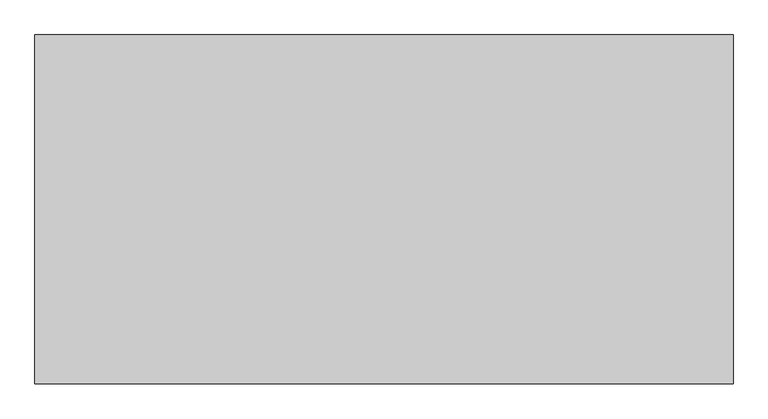
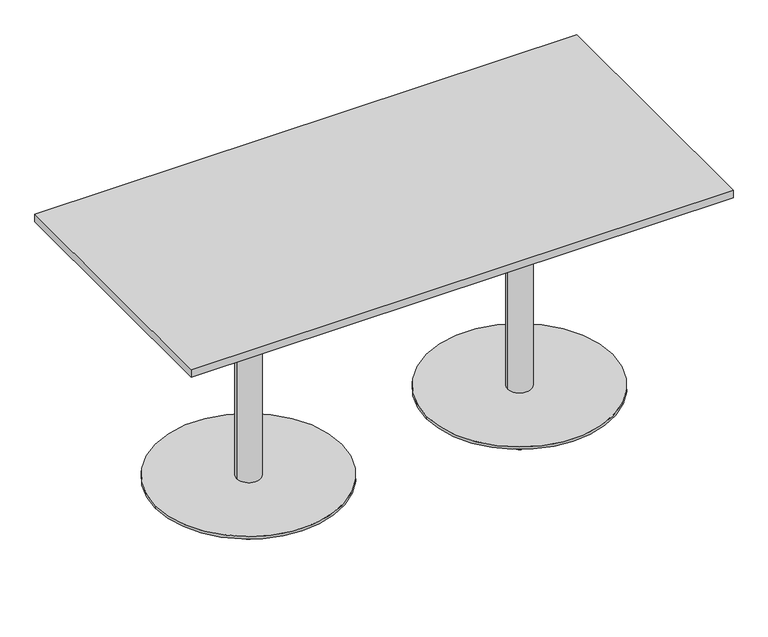
"""IFC4 building model written with IfcOpenShell, lengths in millimetres: furniture geometry, U-MCZZR85N : U-MCZZR85N."""

from ifc_helpers import new_model, si_unit, point, frame, frame_2d, origin, origin_with_axes, place, context, project, spatial, polyline, circle_curve, trimmed, segment, composite_curve, outline, extrude, source, transform, mapped, element, save


def furniture_60f8bc97(model_context):
    return source(origin(), model_context, "Body", "SweptSolid", [
        extrude(outline(composite_curve([segment(trimmed(circle_curve(frame_2d((-655.0001777, 0.0)), 12.5), [point((-667.5001777, 0.0))], [point((-642.5001777, 0.0))], False, "CARTESIAN"), True, "CONTINUOUS"), segment(trimmed(circle_curve(frame_2d((-655.0001777, 0.0)), 12.5), [point((-642.5001777, 0.0))], [point((-667.5001777, 0.0))], False, "CARTESIAN"), True, "CONTINUOUS")], self_intersect=False)), origin_with_axes(), (0.0, 0.0, 1.0), 6.0),
        extrude(outline(composite_curve([segment(trimmed(circle_curve(frame_2d((-527.5000664, 220.835939)), 12.5), [point((-540.0000664, 220.835939))], [point((-515.0000664, 220.835939))], False, "CARTESIAN"), True, "CONTINUOUS"), segment(trimmed(circle_curve(frame_2d((-527.5000664, 220.835939)), 12.5), [point((-515.0000664, 220.835939))], [point((-540.0000664, 220.835939))], False, "CARTESIAN"), True, "CONTINUOUS")], self_intersect=False)), origin_with_axes(), (0.0, 0.0, 1.0), 6.0),
        extrude(outline(composite_curve([segment(trimmed(circle_curve(frame_2d((-272.4999336, 220.835939)), 12.5), [point((-284.9999336, 220.835939))], [point((-259.9999336, 220.835939))], False, "CARTESIAN"), True, "CONTINUOUS"), segment(trimmed(circle_curve(frame_2d((-272.4999336, 220.835939)), 12.5), [point((-259.9999336, 220.835939))], [point((-284.9999336, 220.835939))], False, "CARTESIAN"), True, "CONTINUOUS")], self_intersect=False)), origin_with_axes(), (0.0, 0.0, 1.0), 6.0),
        extrude(outline(composite_curve([segment(trimmed(circle_curve(frame_2d((-144.9998223, 0.0)), 12.5), [point((-157.4998223, 0.0))], [point((-132.4998223, 0.0))], False, "CARTESIAN"), True, "CONTINUOUS"), segment(trimmed(circle_curve(frame_2d((-144.9998223, 0.0)), 12.5), [point((-132.4998223, 0.0))], [point((-157.4998223, 0.0))], False, "CARTESIAN"), True, "CONTINUOUS")], self_intersect=False)), origin_with_axes(), (0.0, 0.0, 1.0), 6.0),
        extrude(outline(composite_curve([segment(trimmed(circle_curve(frame_2d((-527.5000664, -220.835939)), 12.5), [point((-540.0000664, -220.835939))], [point((-515.0000664, -220.835939))], False, "CARTESIAN"), True, "CONTINUOUS"), segment(trimmed(circle_curve(frame_2d((-527.5000664, -220.835939)), 12.5), [point((-515.0000664, -220.835939))], [point((-540.0000664, -220.835939))], False, "CARTESIAN"), True, "CONTINUOUS")], self_intersect=False)), origin_with_axes(), (0.0, 0.0, 1.0), 6.0),
        extrude(outline(composite_curve([segment(trimmed(circle_curve(frame_2d((-272.4999336, -220.835939)), 12.5), [point((-284.9999336, -220.835939))], [point((-259.9999336, -220.835939))], False, "CARTESIAN"), True, "CONTINUOUS"), segment(trimmed(circle_curve(frame_2d((-272.4999336, -220.835939)), 12.5), [point((-259.9999336, -220.835939))], [point((-284.9999336, -220.835939))], False, "CARTESIAN"), True, "CONTINUOUS")], self_intersect=False)), origin_with_axes(), (0.0, 0.0, 1.0), 6.0),
        extrude(outline(composite_curve([segment(trimmed(circle_curve(frame_2d((144.9998223, 0.0)), 12.5), [point((132.4998223, 0.0))], [point((157.4998223, 0.0))], False, "CARTESIAN"), True, "CONTINUOUS"), segment(trimmed(circle_curve(frame_2d((144.9998223, 0.0)), 12.5), [point((157.4998223, 0.0))], [point((132.4998223, 0.0))], False, "CARTESIAN"), True, "CONTINUOUS")], self_intersect=False)), origin_with_axes(), (0.0, 0.0, 1.0), 6.0),
        extrude(outline(composite_curve([segment(trimmed(circle_curve(frame_2d((272.4999336, 220.835939)), 12.5), [point((259.9999336, 220.835939))], [point((284.9999336, 220.835939))], False, "CARTESIAN"), True, "CONTINUOUS"), segment(trimmed(circle_curve(frame_2d((272.4999336, 220.835939)), 12.5), [point((284.9999336, 220.835939))], [point((259.9999336, 220.835939))], False, "CARTESIAN"), True, "CONTINUOUS")], self_intersect=False)), origin_with_axes(), (0.0, 0.0, 1.0), 6.0),
        extrude(outline(composite_curve([segment(trimmed(circle_curve(frame_2d((527.5000664, 220.835939)), 12.5), [point((515.0000664, 220.835939))], [point((540.0000664, 220.835939))], False, "CARTESIAN"), True, "CONTINUOUS"), segment(trimmed(circle_curve(frame_2d((527.5000664, 220.835939)), 12.5), [point((540.0000664, 220.835939))], [point((515.0000664, 220.835939))], False, "CARTESIAN"), True, "CONTINUOUS")], self_intersect=False)), origin_with_axes(), (0.0, 0.0, 1.0), 6.0),
        extrude(outline(composite_curve([segment(trimmed(circle_curve(frame_2d((655.0001777, 0.0)), 12.5), [point((642.5001777, 0.0))], [point((667.5001777, 0.0))], False, "CARTESIAN"), True, "CONTINUOUS"), segment(trimmed(circle_curve(frame_2d((655.0001777, 0.0)), 12.5), [point((667.5001777, 0.0))], [point((642.5001777, 0.0))], False, "CARTESIAN"), True, "CONTINUOUS")], self_intersect=False)), origin_with_axes(), (0.0, 0.0, 1.0), 6.0),
        extrude(outline(composite_curve([segment(trimmed(circle_curve(frame_2d((272.4999336, -220.835939)), 12.5), [point((259.9999336, -220.835939))], [point((284.9999336, -220.835939))], False, "CARTESIAN"), True, "CONTINUOUS"), segment(trimmed(circle_curve(frame_2d((272.4999336, -220.835939)), 12.5), [point((284.9999336, -220.835939))], [point((259.9999336, -220.835939))], False, "CARTESIAN"), True, "CONTINUOUS")], self_intersect=False)), origin_with_axes(), (0.0, 0.0, 1.0), 6.0),
        extrude(outline(composite_curve([segment(trimmed(circle_curve(frame_2d((527.5000664, -220.835939)), 12.5), [point((515.0000664, -220.835939))], [point((540.0000664, -220.835939))], False, "CARTESIAN"), True, "CONTINUOUS"), segment(trimmed(circle_curve(frame_2d((527.5000664, -220.835939)), 12.5), [point((540.0000664, -220.835939))], [point((515.0000664, -220.835939))], False, "CARTESIAN"), True, "CONTINUOUS")], self_intersect=False)), origin_with_axes(), (0.0, 0.0, 1.0), 6.0),
        extrude(outline(composite_curve([segment(trimmed(circle_curve(frame_2d((-400.0, 0.0)), 35.0), [point((-365.0, 0.0))], [point((-435.0, 0.0))], False, "CARTESIAN"), True, "CONTINUOUS"), segment(trimmed(circle_curve(frame_2d((-400.0, 0.0)), 35.0), [point((-435.0, 0.0))], [point((-365.0, 0.0))], False, "CARTESIAN"), True, "CONTINUOUS")], self_intersect=False)), frame((0.0, 0.0, 14.0), z_axis=(0.0, 0.0, 1.0), x_axis=(1.0, 0.0, 0.0)), (0.0, 0.0, 1.0), 688.0),
        extrude(outline(composite_curve([segment(trimmed(circle_curve(frame_2d((400.0, 0.0)), 35.0), [point((435.0, 0.0))], [point((365.0, 0.0))], False, "CARTESIAN"), True, "CONTINUOUS"), segment(trimmed(circle_curve(frame_2d((400.0, 0.0)), 35.0), [point((365.0, 0.0))], [point((435.0, 0.0))], False, "CARTESIAN"), True, "CONTINUOUS")], self_intersect=False)), frame((0.0, 0.0, 14.0), z_axis=(0.0, 0.0, 1.0), x_axis=(1.0, 0.0, 0.0)), (0.0, 0.0, 1.0), 688.0),
        extrude(outline(composite_curve([segment(trimmed(circle_curve(frame_2d((-399.9999834, 0.0)), 275.0), [point((-124.9999834, 0.0))], [point((-674.9999834, 0.0))], False, "CARTESIAN"), True, "CONTINUOUS"), segment(trimmed(circle_curve(frame_2d((-399.9999834, 0.0)), 275.0), [point((-674.9999834, 0.0))], [point((-124.9999834, 0.0))], False, "CARTESIAN"), True, "CONTINUOUS")], self_intersect=False)), frame((0.0, 0.0, 6.0), z_axis=(0.0, 0.0, 1.0), x_axis=(1.0, 0.0, 0.0)), (0.0, 0.0, 1.0), 8.0),
        extrude(outline(composite_curve([segment(trimmed(circle_curve(frame_2d((399.9999834, 0.0)), 275.0), [point((674.9999834, 0.0))], [point((124.9999834, 0.0))], False, "CARTESIAN"), True, "CONTINUOUS"), segment(trimmed(circle_curve(frame_2d((399.9999834, 0.0)), 275.0), [point((124.9999834, 0.0))], [point((674.9999834, 0.0))], False, "CARTESIAN"), True, "CONTINUOUS")], self_intersect=False)), frame((0.0, 0.0, 6.0), z_axis=(0.0, 0.0, 1.0), x_axis=(1.0, 0.0, 0.0)), (0.0, 0.0, 1.0), 8.0),
        extrude(outline(polyline([(800.0, 400.0), (800.0, -400.0), (-800.0, -400.0), (-800.0, 400.0), (800.0, 400.0)])), frame((0.0, 0.0, 702.0), z_axis=(0.0, 0.0, 1.0), x_axis=(1.0, 0.0, 0.0)), (0.0, 0.0, 1.0), 23.0),
    ])


if __name__ == "__main__":
    model = new_model("IFC4")
    model_context = context("Model", 3, world=origin())
    ifc_project = project(units=[si_unit("LENGTHUNIT", "METRE", prefix="MILLI")], contexts=[model_context])
    site = spatial("IfcSite", under=ifc_project)
    building = spatial("IfcBuilding", under=site)
    placement = place(None, origin())
    furniture_shape = furniture_60f8bc97(model_context)
    element("IfcFurniture", 1, ObjectType="U-MCZZR85N : U-MCZZR85N", at=placement, inside=building, context=model_context, shape_type="MappedRepresentation", body=[
        mapped(furniture_shape, transform((0.0, 0.0, 0.0), x_axis=(1.0, 0.0, 0.0), y_axis=(0.0, 1.0, 0.0), z_axis=(0.0, 0.0, 1.0))),
    ])
    save(model, "model.ifc")

# Revit data of these elements
# Type "U-MCZZR85N : U-MCZZR85N"
#   Youtube clip = ""
#   Weight Net (kg) = ""
#   WarrantyStartDate = ""
#   WarrantyDuration = ""
#   Uniclass 2.0 Description = "Desks, Tables And Worktops"
#   Uniclass 2.0 Code = "PR-31-22"
#   Uniclass 1.4 Description = "Conference room furniture"
#   Uniclass 1.4 Code = "L8536"
#   URL = "http://kinnarps.bimobject.com/U-MCZZR85N"
#   UNSPSC Category = "Furniture and Furnishings"
#   TypeName = "U-MCZZR85N"
#   Technical description = "http://www.kinnarps.com/en/International/ProductsInspiration/Office/ConferenceTables/Product/?prodid=305786"
#   TagNumber = ""
#   Size = ""
#   SerialNumber = ""
#   Product identifier = "kinnarps.bimobject.com/U-MCZZR85N"
#   Product group = "MULTICOM"
#   Product family = "Conference tables"
#   Product data url = "http://www.kinnarps.com/en/International/ProductsInspiration/Office/ConferenceTables/Product/?prodid=305786"
#   Product SKU = "U-MCZZR85N"
#   Omniclass = "23.40.70.14.64.11"
#   NominalWidth = ""
#   NominalHeight = ""
#   Name of the object = "MULTICOM U-MCZZR85N"
#   NBS Reference Description = "Desks, Tables And Worktops"
#   NBS Reference = "31-22"
#   Model = "MULTICOM U-MCZZR85N"
#   Material = ""
#   Manufacturer country = "Sweden"
#   Manufacturer URL = "http://www.kinnarps.com"
#   Manufacturer = "Kinnarps"
#   InstallationDate = ""
#   Installation instructions = "http://www.kinnarps.com/en/International/ProductsInspiration/Office/ConferenceTables/Product/?prodid=305786"
#   IFC Classification = "Furniture"
#   Grade = ""
#   Finish = ""
#   Features = ""
#   Extidentifier = ""
#   Edition number = "1"
#   EAN code = ""
#   Design country = "Sweden"
#   Date of publishing = ""
#   Created on = ""
#   Created by = ""
#   ConnectionType = ""
#   Colour = ""
#   COBIe Type Category = ""
#   Barcode = ""
#   BIMobject QR code url = "http://kinnarps.bimobject.com/U-MCZZR85N"
#   BIMobject Category = "Office Furniture"
#   AssetIdentifier = ""
#   AccessibilityPerformance = ""
#   Y-Offset = 0 mm
#   Width (mm) = 1600 mm
#   X-Offset = 0 mm
#   Height (mm) = 725 mm
#   Depth (mm) = 800 mm
#   UNSPSC Code = 56
#   Table Top [instance default] = Kinnarps-Laminate-Beech
#   Table Leg [instance default] = Kinnarps-Metal-White
#   Material secondary = Steel
#   Material main = Laminate, Linen, Matte
#   Default Elevation = 0
# Element 1 (IfcFurniture, "U-MCZZR85N : U-MCZZR85N")
#   Table Top = Kinnarps-Laminate-White
#   Table Leg = Kinnarps-Metal-Silver
#   Materials on its faces: "Kinnarps-Plastic-Black", "Kinnarps-Metal-Silver", "Kinnarps-Laminate-White"
# Materials
#   "Kinnarps-Laminate-Beech": class "Miscellaneous", colour RGB 174 140 106, transparency 0
#   "Kinnarps-Metal-White": class "Miscellaneous", colour RGB 255 255 255, transparency 0
#   "Steel": class "Metal", colour RGB 189 187 185, transparency 0, Cost = 0
#   "Laminate, Linen, Matte": class "Plastic", colour RGB 198 189 176, transparency 0, Description = "Plastic Laminate - Linen, Matte", Cost = 0
#   "Kinnarps-Plastic-Black": class "Miscellaneous", colour RGB 0 0 0, transparency 0
#   "Kinnarps-Metal-Silver": class "Miscellaneous", colour RGB 168 168 168, transparency 0
#   "Kinnarps-Laminate-White": class "Miscellaneous", colour RGB 255 255 255, transparency 0
